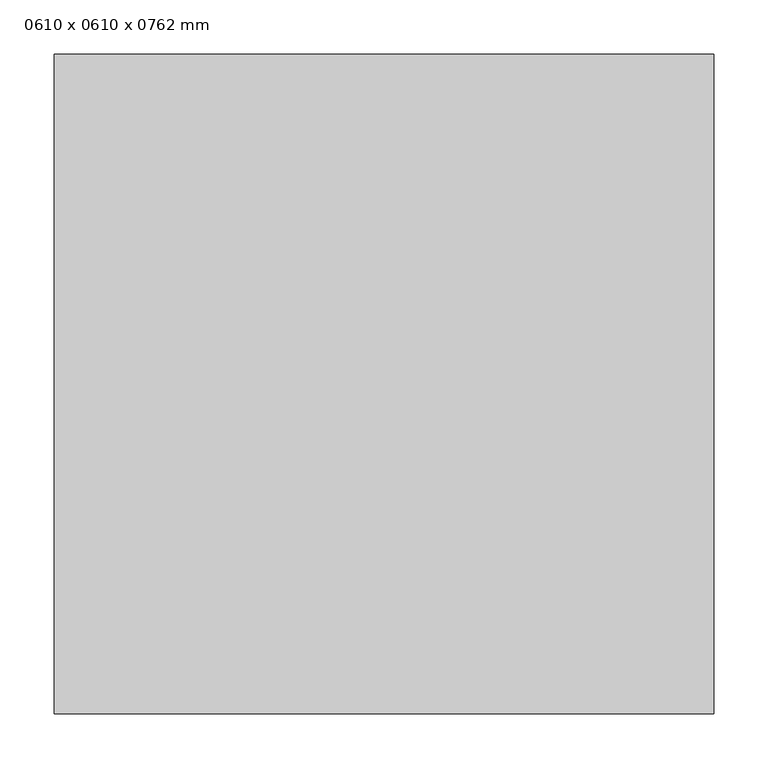
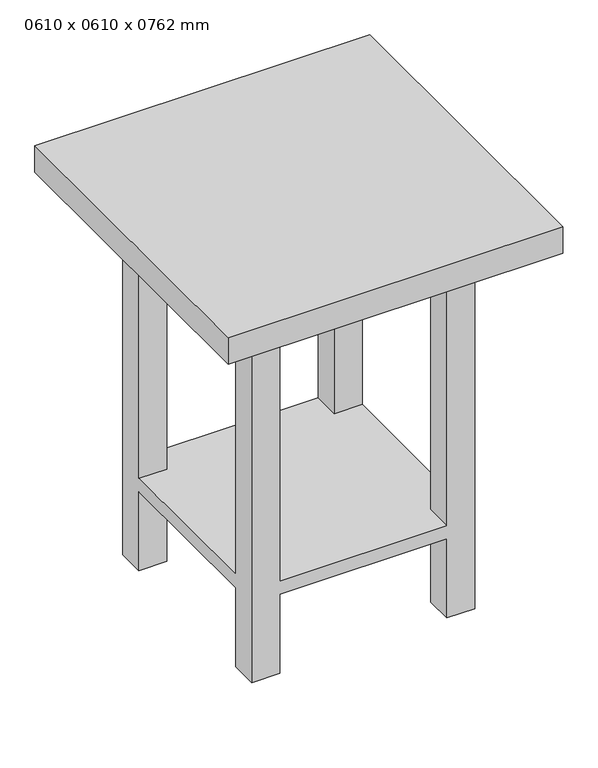
"""IFC4 building model written with IfcOpenShell, lengths in millimetres: furniture geometry, Mesa-Mesita de noche : 0610 x 0610 x 0762 mm."""

from ifc_helpers import new_model, si_unit, frame, origin, place, context, project, spatial, polyline, outline, extrude, faceted_brep, source, transform, mapped, element, save


def furniture_0610_x_0610_x_0762_mm_a39a3fb5(model_context):
    return source(origin(), model_context, "Body", "SolidModel", [
        faceted_brep([(156.1336303, 508.4, 711.2), (105.3336303, 508.4, 711.2), (105.3336303, 457.6, 711.2), (156.1336303, 457.6, 711.2), (156.1336303, 152.4, 711.2), (105.3336303, 152.4, 711.2), (105.3336303, 101.6, 711.2), (156.1336303, 101.6, 711.2), (512.1336303, 508.4, 711.2), (461.3336303, 508.4, 711.2), (461.3336303, 457.6, 711.2), (512.1336303, 457.6, 711.2), (512.1336303, 152.4, 711.2), (461.3336303, 152.4, 711.2), (461.3336303, 101.6, 711.2), (512.1336303, 101.6, 711.2), (156.1336303, 508.4, 0.0), (156.1336303, 457.6, 0.0), (105.3336303, 457.6, 0.0), (105.3336303, 508.4, 0.0), (156.1336303, 152.4, 0.0), (156.1336303, 101.6, 0.0), (105.3336303, 101.6, 0.0), (105.3336303, 152.4, 0.0), (512.1336303, 508.4, 0.0), (512.1336303, 457.6, 0.0), (461.3336303, 457.6, 0.0), (461.3336303, 508.4, 0.0), (512.1336303, 152.4, 0.0), (512.1336303, 101.6, 0.0), (461.3336303, 101.6, 0.0), (461.3336303, 152.4, 0.0), (156.1336303, 508.4, 177.8), (461.3336303, 508.4, 177.8), (461.3336303, 508.4, 152.4), (156.1336303, 508.4, 152.4), (105.3336303, 457.6, 152.4), (105.3336303, 152.4, 152.4), (105.3336303, 152.4, 177.8), (105.3336303, 457.6, 177.8), (156.1336303, 457.6, 177.8), (156.1336303, 457.6, 152.4), (156.1336303, 152.4, 177.8), (156.1336303, 152.4, 152.4), (156.1336303, 101.6, 152.4), (461.3336303, 101.6, 152.4), (461.3336303, 101.6, 177.8), (156.1336303, 101.6, 177.8), (461.3336303, 457.6, 177.8), (461.3336303, 457.6, 152.4), (512.1336303, 457.6, 177.8), (512.1336303, 457.6, 152.4), (512.1336303, 152.4, 177.8), (512.1336303, 152.4, 152.4), (461.3336303, 152.4, 177.8), (461.3336303, 152.4, 152.4)], [[[0, 1, 2, 3]], [[4, 5, 6, 7]], [[8, 9, 10, 11]], [[12, 13, 14, 15]], [[16, 17, 18, 19]], [[20, 21, 22, 23]], [[24, 25, 26, 27]], [[28, 29, 30, 31]], [[1, 0, 32, 33, 9, 8, 24, 27, 34, 35, 16, 19]], [[2, 1, 19, 18, 36, 37, 23, 22, 6, 5, 38, 39]], [[3, 2, 39, 40]], [[18, 17, 41, 36]], [[0, 3, 40, 32]], [[17, 16, 35, 41]], [[5, 4, 42, 38]], [[20, 23, 37, 43]], [[7, 6, 22, 21, 44, 45, 30, 29, 15, 14, 46, 47]], [[4, 7, 47, 42]], [[21, 20, 43, 44]], [[10, 9, 33, 48]], [[27, 26, 49, 34]], [[11, 10, 48, 50]], [[26, 25, 51, 49]], [[8, 11, 50, 52, 12, 15, 29, 28, 53, 51, 25, 24]], [[13, 12, 52, 54]], [[28, 31, 55, 53]], [[14, 13, 54, 46]], [[31, 30, 45, 55]], [[39, 38, 42, 47, 46, 54, 52, 50, 48, 33, 32, 40]], [[35, 34, 49, 51, 53, 55, 45, 44, 43, 37, 36, 41]]]),
        extrude(outline(polyline([(613.7336303, 0.0), (3.7336303, 0.0), (3.7336303, 610.0), (613.7336303, 610.0), (613.7336303, 0.0)])), frame((0.0, 0.0, 711.2), z_axis=(0.0, 0.0, 1.0), x_axis=(1.0, 0.0, 0.0)), (0.0, 0.0, 1.0), 50.8),
    ])


if __name__ == "__main__":
    model = new_model("IFC4")
    model_context = context("Model", 3, world=origin())
    ifc_project = project(units=[si_unit("LENGTHUNIT", "METRE", prefix="MILLI")], contexts=[model_context])
    site = spatial("IfcSite", under=ifc_project)
    building = spatial("IfcBuilding", under=site)
    placement = place(None, origin())
    furniture_0610_x_0610_x_0762_mm_shape = furniture_0610_x_0610_x_0762_mm_a39a3fb5(model_context)
    element("IfcFurniture", 1, ObjectType="Mesa-Mesita de noche : 0610 x 0610 x 0762 mm", at=placement, inside=building, context=model_context, shape_type="MappedRepresentation", body=[
        mapped(furniture_0610_x_0610_x_0762_mm_shape, transform((0.0, 0.0, 0.0), x_axis=(1.0, 0.0, 0.0), y_axis=(0.0, 1.0, 0.0), z_axis=(0.0, 0.0, 1.0))),
    ])
    save(model, "model.ifc")

# Revit data of these elements
# Type "Mesa-Mesita de noche : 0610 x 0610 x 0762 mm"
#   Profundidad = 0.61 m
#   Altura = 0.762 m
#   Anchura = 0.61 m
#   Máscara [instance default] = yes
#   Material base = Madera - Abedul
#   Material de parte superior = Laminado - Marfil, Mate
#   Default Elevation = 0
# Element 1 (IfcFurniture, "Mesa-Mesita de noche : 0610 x 0610 x 0762 mm")
#   Materials on its faces: "Madera - Abedul", "Laminado - Marfil, Mate"
# Materials
#   "Madera - Abedul": class "Madera", colour RGB 224 178 126, transparency 0
#   "Laminado - Marfil, Mate": class "Varios", colour RGB 247 247 239, transparency 0
